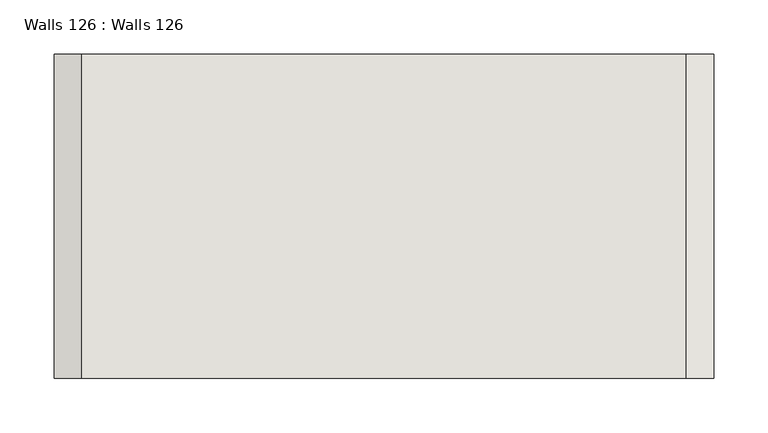
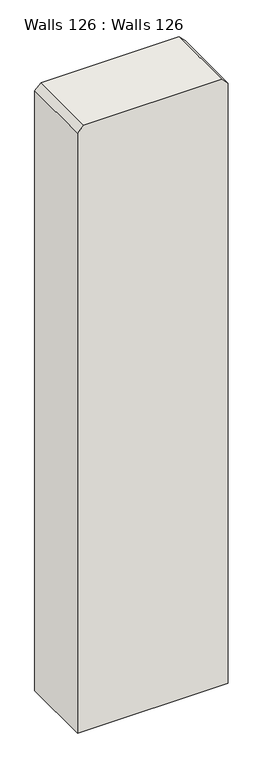
"""IFC4 building model written with IfcOpenShell, lengths in millimetres: wall geometry, Walls 126 : Walls 126."""

import ifcopenshell
import ifcopenshell.guid

model = None  # the IFC model being written
_history = None  # IfcOwnerHistory: only IFC2X3 demands one
_inside = {}  # id of a spatial element -> (the spatial element, [elements in it])
_under = {}  # id of a project, library or spatial element -> (it, [spatial elements below it])
_declared = {}  # id of a project -> (the project, [libraries it declares])
_typed = {}  # id of a type object -> (the type object, [elements of that type])
_made_of = {}  # id of a material, layer set ... -> (it, [elements and type objects made of it])


def new_model(schema):
    """Start an empty IFC model of exactly this schema.

    Asked for "IFC4X3", IfcOpenShell would pick the latest addendum, in which some entities
    have other attributes; the version numbers below select the first issue.
    IFC2X3 requires an IfcOwnerHistory on every rooted entity: one is made here for all.
    """
    global model, _history
    if schema == "IFC4X3":
        model = ifcopenshell.file(schema_version=(4, 3, 0, 0))
    else:
        model = ifcopenshell.file(schema=schema)
    _inside.clear()
    _under.clear()
    _declared.clear()
    _typed.clear()
    _made_of.clear()
    _history = None
    if model.schema == "IFC2X3":
        org = make("IfcOrganization", Name="unknown")
        user = make(
            "IfcPersonAndOrganization",
            ThePerson=make("IfcPerson", FamilyName="unknown"),
            TheOrganization=org,
        )
        app = make(
            "IfcApplication",
            ApplicationDeveloper=org,
            Version="unknown",
            ApplicationFullName="unknown",
            ApplicationIdentifier="unknown",
        )
        _history = make(
            "IfcOwnerHistory",
            OwningUser=user,
            OwningApplication=app,
            ChangeAction="ADDED",
            CreationDate=0,
        )
    return model


def make(cls, **values):
    """One entity of the class cls with the attributes given. An attribute that is None is left unset."""
    return model.create_entity(
        cls, **{name: value for name, value in values.items() if value is not None}
    )


def rooted(cls, **values):
    """An entity with a GlobalId (a new one), such as an element, a storey or a relation."""
    return make(cls, GlobalId=ifcopenshell.guid.new(), OwnerHistory=_history, **values)


def si_unit(unit_type, name, prefix=None):
    """IfcSIUnit, for example si_unit("LENGTHUNIT", "METRE", prefix="MILLI")."""
    return make("IfcSIUnit", UnitType=unit_type, Prefix=prefix, Name=name)


def assignment(units):
    """IfcUnitAssignment: the units of a project."""
    return None if units is None else make("IfcUnitAssignment", Units=units)


def point(xyz):
    """IfcCartesianPoint."""
    return None if xyz is None else make("IfcCartesianPoint", Coordinates=xyz)


def direction(xyz):
    """IfcDirection."""
    return None if xyz is None else make("IfcDirection", DirectionRatios=xyz)


def frame(location, z_axis=None, x_axis=None):
    """IfcAxis2Placement3D, a coordinate frame: its origin and axes. An axis left out is left unset."""
    return make(
        "IfcAxis2Placement3D",
        Location=point(location),
        Axis=direction(z_axis),
        RefDirection=direction(x_axis),
    )


def origin():
    """The frame at (0, 0, 0) with its axes left unset."""
    return frame((0.0, 0.0, 0.0))


def place(relative_to, where):
    """IfcLocalPlacement: puts the frame where relative to a parent placement (None: the world)."""
    return make(
        "IfcLocalPlacement", PlacementRelTo=relative_to, RelativePlacement=where
    )


def context(
    kind, dimensions, precision=None, world=None, true_north=None, identifier=None
):
    """IfcGeometricRepresentationContext, for example the 3D "Model" context."""
    return make(
        "IfcGeometricRepresentationContext",
        ContextIdentifier=identifier,
        ContextType=kind,
        CoordinateSpaceDimension=dimensions,
        Precision=precision,
        WorldCoordinateSystem=world,
        TrueNorth=true_north,
    )


def project(units=None, contexts=None):
    """IfcProject with its units and contexts."""
    return rooted(
        "IfcProject",
        Name="project",
        RepresentationContexts=contexts,
        UnitsInContext=assignment(units),
    )


def spatial(cls, under=None, at=None, **own):
    """A site, building, storey or space (cls), placed at a placement, below another one or the project."""
    s = rooted(cls, ObjectPlacement=at, **own)
    if under is not None:
        _under.setdefault(under.id(), (under, []))[1].append(s)
    return s


def polyline(points):
    """IfcPolyline through the points."""
    return make("IfcPolyline", Points=[point(p) for p in points])


def outline(outer, holes=None, kind="AREA"):
    """IfcArbitraryClosedProfileDef: a profile drawn as a closed curve; with holes, ...WithVoids."""
    if holes is None:
        return make("IfcArbitraryClosedProfileDef", ProfileType=kind, OuterCurve=outer)
    return make(
        "IfcArbitraryProfileDefWithVoids",
        ProfileType=kind,
        OuterCurve=outer,
        InnerCurves=holes,
    )


def extrude(swept, where, along, depth):
    """IfcExtrudedAreaSolid: the profile swept, set in the frame where, extruded along a direction by depth."""
    return make(
        "IfcExtrudedAreaSolid",
        SweptArea=swept,
        Position=where,
        ExtrudedDirection=direction(along),
        Depth=depth,
    )


def shape(context_of_items, identifier, shape_type, items):
    """IfcShapeRepresentation: the items that make up one representation, for example the "Body"."""
    return make(
        "IfcShapeRepresentation",
        ContextOfItems=context_of_items,
        RepresentationIdentifier=identifier,
        RepresentationType=shape_type,
        Items=items,
    )


def source(mapping_origin, context_of_items, identifier, shape_type, items):
    """IfcRepresentationMap: a shape defined once, which mapped items show again and again."""
    return make(
        "IfcRepresentationMap",
        MappingOrigin=mapping_origin,
        MappedRepresentation=shape(context_of_items, identifier, shape_type, items),
    )


def transform(
    local_origin,
    x_axis=None,
    y_axis=None,
    z_axis=None,
    scale=None,
    scale2=None,
    scale3=None,
    uniform=True,
):
    """IfcCartesianTransformationOperator3D, or its non-uniform kind. x_axis, y_axis, z_axis: its Axis1, 2, 3."""
    if uniform:
        return make(
            "IfcCartesianTransformationOperator3D",
            Axis1=direction(x_axis),
            Axis2=direction(y_axis),
            LocalOrigin=point(local_origin),
            Scale=scale,
            Axis3=direction(z_axis),
        )
    return make(
        "IfcCartesianTransformationOperator3DnonUniform",
        Axis1=direction(x_axis),
        Axis2=direction(y_axis),
        LocalOrigin=point(local_origin),
        Scale=scale,
        Axis3=direction(z_axis),
        Scale2=scale2,
        Scale3=scale3,
    )


def mapped(mapping_source, mapping_target):
    """IfcMappedItem: shows the shape of a source again, moved by a transform."""
    return make(
        "IfcMappedItem", MappingSource=mapping_source, MappingTarget=mapping_target
    )


def made_of(thing, what):
    """Note that an element or type object is made of a material, layer set ...; save() writes the relation."""
    if what is not None:
        _made_of.setdefault(what.id(), (what, []))[1].append(thing)
    return thing


def element(
    cls,
    number,
    at=None,
    inside=None,
    cuts=None,
    type_object=None,
    material=None,
    context=None,
    identifier="Body",
    shape_type=None,
    held_by="IfcProductDefinitionShape",
    body=None,
    shapes=None,
    **own,
):
    """One element of the class cls, such as IfcWall. Its Tag is "e" and its number.

    at: its placement. inside: the storey or other place that contains it. cuts: it is an
    opening in that element (IfcRelVoidsElement). A single representation is given by context,
    identifier, shape_type and body (its items); several are given by shapes. held_by: the class
    of the entity that holds the representations. save() writes the other relations.
    """
    e = rooted(cls, Tag="e%d" % number, ObjectPlacement=at, **own)
    if body is not None:
        shapes = [shape(context, identifier, shape_type, body)]
    if shapes is not None:
        e.Representation = make(held_by, Representations=shapes)
    if inside is not None:
        _inside.setdefault(inside.id(), (inside, []))[1].append(e)
    if cuts is not None:
        rooted(
            "IfcRelVoidsElement", RelatingBuildingElement=cuts, RelatedOpeningElement=e
        )
    if type_object is not None:
        _typed.setdefault(type_object.id(), (type_object, []))[1].append(e)
    return made_of(e, material)


def aggregate(whole, parts):
    """IfcRelAggregates: a whole, such as a stair, and the parts it consists of."""
    return rooted("IfcRelAggregates", RelatingObject=whole, RelatedObjects=parts)


def save(model, path):
    """Write the relations noted so far, then the file.

    IfcRelAggregates (storeys below a building ...), IfcRelContainedInSpatialStructure (elements
    in a storey), IfcRelDefinesByType, IfcRelAssociatesMaterial and IfcRelDeclares: one each for
    every whole, place, type object, material and project.
    """
    for whole, parts in _under.values():
        aggregate(whole, parts)
    for where, things in _inside.values():
        rooted(
            "IfcRelContainedInSpatialStructure",
            RelatedElements=things,
            RelatingStructure=where,
        )
    for kind, things in _typed.values():
        rooted("IfcRelDefinesByType", RelatedObjects=things, RelatingType=kind)
    for what, things in _made_of.values():
        rooted("IfcRelAssociatesMaterial", RelatedObjects=things, RelatingMaterial=what)
    for by, libraries in _declared.values():
        rooted("IfcRelDeclares", RelatingContext=by, RelatedDefinitions=libraries)
    model.write(path)


def walls_126_walls_126_7fe6290c(model_context):
    return source(origin(), model_context, "Body", "SweptSolid", [
        extrude(outline(polyline([(111.2346173, 39644.9681437), (2676.6346173, 39644.9681437), (2702.0346173, 39619.5681437), (2702.0346173, 39060.7681437), (2676.6346173, 39035.3681437), (111.2346173, 39035.3681437), (111.2346173, 39644.9681437)])), frame((0.0, 613.3825707, 0.0), z_axis=(0.0, 1.0, 0.0), x_axis=(0.0, 0.0, 1.0)), (0.0, 0.0, 1.0), 299.3524407),
    ])


if __name__ == "__main__":
    model = new_model("IFC4")
    model_context = context("Model", 3, world=origin())
    ifc_project = project(units=[si_unit("LENGTHUNIT", "METRE", prefix="MILLI")], contexts=[model_context])
    site = spatial("IfcSite", under=ifc_project)
    building = spatial("IfcBuilding", under=site)
    placement = place(None, origin())
    walls_126_walls_126_shape = walls_126_walls_126_7fe6290c(model_context)
    element("IfcWall", 1, ObjectType="Walls 126 : Walls 126", at=placement, inside=building, context=model_context, shape_type="MappedRepresentation", body=[
        mapped(walls_126_walls_126_shape, transform((0.0, 0.0, 0.0), x_axis=(1.0, 0.0, 0.0), y_axis=(0.0, 1.0, 0.0), z_axis=(0.0, 0.0, 1.0))),
    ])
    save(model, "model.ifc")

# Revit data of these elements
# Element 1 (IfcWall, "Walls 126 : Walls 126")
#   Materials on its faces: "24\" DIA. CONCRETE POLE BASE WITH THOROSEAL FINISH"
# Materials
#   "24\" DIA. CONCRETE POLE BASE WITH THOROSEAL FINISH": class "Concrete", colour RGB 191 191 191, transparency 0, Description = "Lightweight concrete", Cost = 0
